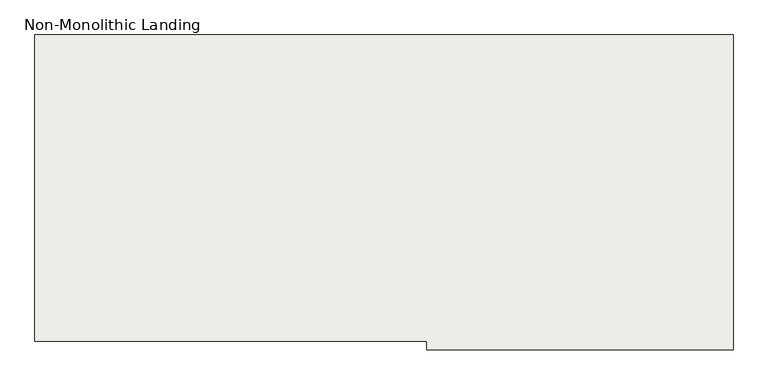
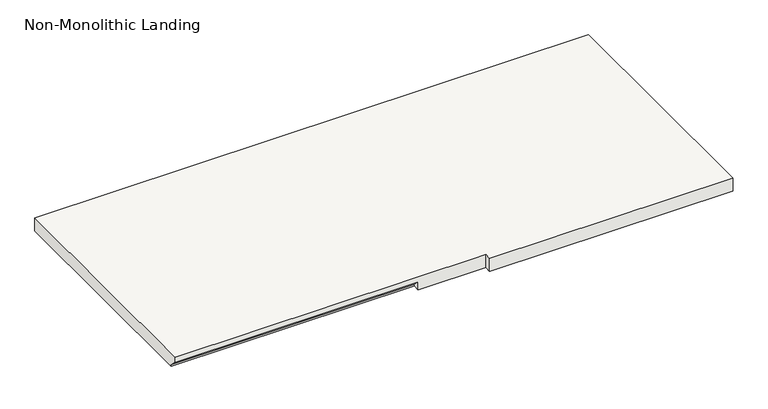
"""IFC4 building model written with IfcOpenShell, lengths in millimetres: slab geometry, Non-Monolithic Landing."""

from ifc_helpers import new_model, si_unit, origin, place, context, project, spatial, faceted_brep, source, transform, mapped, element, save


def non_monolithic_landing_ca5ed38c(model_context):
    return source(origin(), model_context, "Body", "Brep", [
        faceted_brep([(14913.1123343, 17121.2483822, 1504.95), (14913.1123343, 17146.6483822, 1479.55), (15827.5123343, 17146.6483822, 1479.55), (15827.5123343, 17121.2483822, 1504.95), (16081.5123343, 17121.2483822, 1524.0), (16081.5123343, 17095.8483822, 1524.0), (16995.9123343, 17095.8483822, 1524.0), (16995.9123343, 17121.2483822, 1524.0), (16995.9123343, 18035.6483822, 1524.0), (14913.1123343, 18035.6483822, 1524.0), (14913.1123343, 17121.2483822, 1524.0), (15827.5123343, 17146.6483822, 1473.2), (14913.1123343, 17146.6483822, 1473.2), (14913.1123343, 18035.6483822, 1473.2), (16995.9123343, 18035.6483822, 1473.2), (16995.9123343, 17121.2483822, 1473.2), (16995.9123343, 17095.8483822, 1473.2), (16081.5123343, 17095.8483822, 1473.2), (16081.5123343, 17121.2483822, 1473.2), (15827.5123343, 17121.2483822, 1473.2)], [[[0, 1, 2, 3]], [[4, 5, 6, 7, 8, 9, 10]], [[11, 12, 13, 14, 15, 16, 17, 18, 19]], [[12, 11, 2, 1]], [[11, 19, 3, 2]], [[4, 10, 0, 3, 19, 18]], [[5, 4, 18, 17]], [[6, 5, 17, 16]], [[7, 6, 16, 15]], [[8, 7, 15, 14]], [[9, 8, 14, 13]], [[10, 9, 13, 12, 1, 0]]]),
    ])


if __name__ == "__main__":
    model = new_model("IFC4")
    model_context = context("Model", 3, world=origin())
    ifc_project = project(units=[si_unit("LENGTHUNIT", "METRE", prefix="MILLI")], contexts=[model_context])
    site = spatial("IfcSite", under=ifc_project)
    building = spatial("IfcBuilding", under=site)
    placement = place(None, origin())
    non_monolithic_landing_shape = non_monolithic_landing_ca5ed38c(model_context)
    element("IfcSlab", 1, ObjectType="Non-Monolithic Landing", at=placement, inside=building, context=model_context, shape_type="MappedRepresentation", body=[
        mapped(non_monolithic_landing_shape, transform((0.0, 0.0, 0.0), x_axis=(1.0, 0.0, 0.0), y_axis=(0.0, 1.0, 0.0), z_axis=(0.0, 0.0, 1.0))),
    ])
    save(model, "model.ifc")
